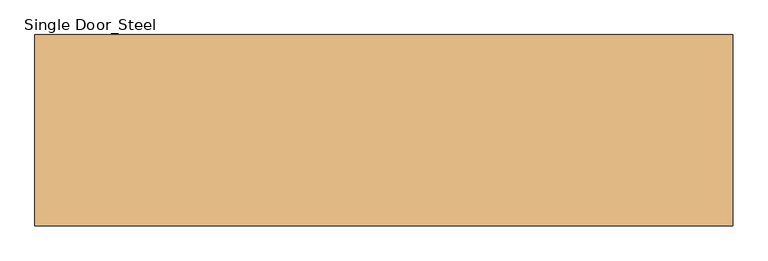
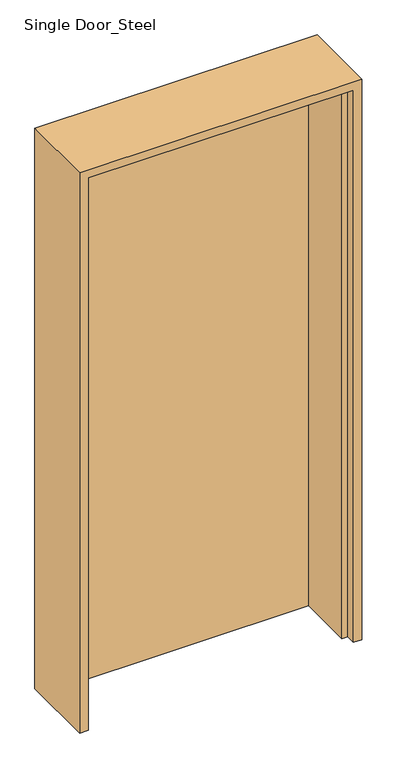
"""IFC4 building model written with IfcOpenShell, lengths in millimetres: door geometry, Single Door_Steel : H_DR_AMD_Single Door_Int_Steel_1000x2100."""

import ifcopenshell
import ifcopenshell.guid

model = None  # the IFC model being written
_history = None  # IfcOwnerHistory: only IFC2X3 demands one
_inside = {}  # id of a spatial element -> (the spatial element, [elements in it])
_under = {}  # id of a project, library or spatial element -> (it, [spatial elements below it])
_declared = {}  # id of a project -> (the project, [libraries it declares])
_typed = {}  # id of a type object -> (the type object, [elements of that type])
_made_of = {}  # id of a material, layer set ... -> (it, [elements and type objects made of it])


def new_model(schema):
    """Start an empty IFC model of exactly this schema.

    Asked for "IFC4X3", IfcOpenShell would pick the latest addendum, in which some entities
    have other attributes; the version numbers below select the first issue.
    IFC2X3 requires an IfcOwnerHistory on every rooted entity: one is made here for all.
    """
    global model, _history
    if schema == "IFC4X3":
        model = ifcopenshell.file(schema_version=(4, 3, 0, 0))
    else:
        model = ifcopenshell.file(schema=schema)
    _inside.clear()
    _under.clear()
    _declared.clear()
    _typed.clear()
    _made_of.clear()
    _history = None
    if model.schema == "IFC2X3":
        org = make("IfcOrganization", Name="unknown")
        user = make(
            "IfcPersonAndOrganization",
            ThePerson=make("IfcPerson", FamilyName="unknown"),
            TheOrganization=org,
        )
        app = make(
            "IfcApplication",
            ApplicationDeveloper=org,
            Version="unknown",
            ApplicationFullName="unknown",
            ApplicationIdentifier="unknown",
        )
        _history = make(
            "IfcOwnerHistory",
            OwningUser=user,
            OwningApplication=app,
            ChangeAction="ADDED",
            CreationDate=0,
        )
    return model


def make(cls, **values):
    """One entity of the class cls with the attributes given. An attribute that is None is left unset."""
    return model.create_entity(
        cls, **{name: value for name, value in values.items() if value is not None}
    )


def rooted(cls, **values):
    """An entity with a GlobalId (a new one), such as an element, a storey or a relation."""
    return make(cls, GlobalId=ifcopenshell.guid.new(), OwnerHistory=_history, **values)


def si_unit(unit_type, name, prefix=None):
    """IfcSIUnit, for example si_unit("LENGTHUNIT", "METRE", prefix="MILLI")."""
    return make("IfcSIUnit", UnitType=unit_type, Prefix=prefix, Name=name)


def assignment(units):
    """IfcUnitAssignment: the units of a project."""
    return None if units is None else make("IfcUnitAssignment", Units=units)


def point(xyz):
    """IfcCartesianPoint."""
    return None if xyz is None else make("IfcCartesianPoint", Coordinates=xyz)


def direction(xyz):
    """IfcDirection."""
    return None if xyz is None else make("IfcDirection", DirectionRatios=xyz)


def frame(location, z_axis=None, x_axis=None):
    """IfcAxis2Placement3D, a coordinate frame: its origin and axes. An axis left out is left unset."""
    return make(
        "IfcAxis2Placement3D",
        Location=point(location),
        Axis=direction(z_axis),
        RefDirection=direction(x_axis),
    )


def origin():
    """The frame at (0, 0, 0) with its axes left unset."""
    return frame((0.0, 0.0, 0.0))


def origin_with_axes():
    """The frame at (0, 0, 0) with the z axis (0, 0, 1) and the x axis (1, 0, 0) written out."""
    return frame((0.0, 0.0, 0.0), z_axis=(0.0, 0.0, 1.0), x_axis=(1.0, 0.0, 0.0))


def place(relative_to, where):
    """IfcLocalPlacement: puts the frame where relative to a parent placement (None: the world)."""
    return make(
        "IfcLocalPlacement", PlacementRelTo=relative_to, RelativePlacement=where
    )


def context(
    kind, dimensions, precision=None, world=None, true_north=None, identifier=None
):
    """IfcGeometricRepresentationContext, for example the 3D "Model" context."""
    return make(
        "IfcGeometricRepresentationContext",
        ContextIdentifier=identifier,
        ContextType=kind,
        CoordinateSpaceDimension=dimensions,
        Precision=precision,
        WorldCoordinateSystem=world,
        TrueNorth=true_north,
    )


def project(units=None, contexts=None):
    """IfcProject with its units and contexts."""
    return rooted(
        "IfcProject",
        Name="project",
        RepresentationContexts=contexts,
        UnitsInContext=assignment(units),
    )


def spatial(cls, under=None, at=None, **own):
    """A site, building, storey or space (cls), placed at a placement, below another one or the project."""
    s = rooted(cls, ObjectPlacement=at, **own)
    if under is not None:
        _under.setdefault(under.id(), (under, []))[1].append(s)
    return s


def polyline(points):
    """IfcPolyline through the points."""
    return make("IfcPolyline", Points=[point(p) for p in points])


def outline(outer, holes=None, kind="AREA"):
    """IfcArbitraryClosedProfileDef: a profile drawn as a closed curve; with holes, ...WithVoids."""
    if holes is None:
        return make("IfcArbitraryClosedProfileDef", ProfileType=kind, OuterCurve=outer)
    return make(
        "IfcArbitraryProfileDefWithVoids",
        ProfileType=kind,
        OuterCurve=outer,
        InnerCurves=holes,
    )


def extrude(swept, where, along, depth):
    """IfcExtrudedAreaSolid: the profile swept, set in the frame where, extruded along a direction by depth."""
    return make(
        "IfcExtrudedAreaSolid",
        SweptArea=swept,
        Position=where,
        ExtrudedDirection=direction(along),
        Depth=depth,
    )


def faces_of(points, faces, orient=None, outer=None):
    """IfcFace entities. A face is a list of loops; a loop is a list of indices into points, from 0.

    orient and outer hold one flag for each loop. By default every Orientation is true, the
    first loop of a face is its IfcFaceOuterBound and the others are IfcFaceBound.
    """
    made = []
    for i, loops in enumerate(faces):
        bounds = []
        for j, loop in enumerate(loops):
            is_outer = j == 0 if outer is None else outer[i][j]
            bounds.append(
                make(
                    "IfcFaceOuterBound" if is_outer else "IfcFaceBound",
                    Bound=make("IfcPolyLoop", Polygon=[points[k] for k in loop]),
                    Orientation=True if orient is None else orient[i][j],
                )
            )
        made.append(make("IfcFace", Bounds=bounds))
    return made


def faceted_brep(points, faces, orient=None, outer=None, voids=None):
    """IfcFacetedBrep: a solid bounded by flat faces; with voids (closed shells), ...WithVoids."""
    shared = [point(p) for p in points]
    hull = make("IfcClosedShell", CfsFaces=faces_of(shared, faces, orient, outer))
    if voids is None:
        return make("IfcFacetedBrep", Outer=hull)
    return make(
        "IfcFacetedBrepWithVoids",
        Outer=hull,
        Voids=[
            make(cls, CfsFaces=faces_of(shared, fs, o, b)) for cls, fs, o, b in voids
        ],
    )


def shape(context_of_items, identifier, shape_type, items):
    """IfcShapeRepresentation: the items that make up one representation, for example the "Body"."""
    return make(
        "IfcShapeRepresentation",
        ContextOfItems=context_of_items,
        RepresentationIdentifier=identifier,
        RepresentationType=shape_type,
        Items=items,
    )


def source(mapping_origin, context_of_items, identifier, shape_type, items):
    """IfcRepresentationMap: a shape defined once, which mapped items show again and again."""
    return make(
        "IfcRepresentationMap",
        MappingOrigin=mapping_origin,
        MappedRepresentation=shape(context_of_items, identifier, shape_type, items),
    )


def transform(
    local_origin,
    x_axis=None,
    y_axis=None,
    z_axis=None,
    scale=None,
    scale2=None,
    scale3=None,
    uniform=True,
):
    """IfcCartesianTransformationOperator3D, or its non-uniform kind. x_axis, y_axis, z_axis: its Axis1, 2, 3."""
    if uniform:
        return make(
            "IfcCartesianTransformationOperator3D",
            Axis1=direction(x_axis),
            Axis2=direction(y_axis),
            LocalOrigin=point(local_origin),
            Scale=scale,
            Axis3=direction(z_axis),
        )
    return make(
        "IfcCartesianTransformationOperator3DnonUniform",
        Axis1=direction(x_axis),
        Axis2=direction(y_axis),
        LocalOrigin=point(local_origin),
        Scale=scale,
        Axis3=direction(z_axis),
        Scale2=scale2,
        Scale3=scale3,
    )


def mapped(mapping_source, mapping_target):
    """IfcMappedItem: shows the shape of a source again, moved by a transform."""
    return make(
        "IfcMappedItem", MappingSource=mapping_source, MappingTarget=mapping_target
    )


def made_of(thing, what):
    """Note that an element or type object is made of a material, layer set ...; save() writes the relation."""
    if what is not None:
        _made_of.setdefault(what.id(), (what, []))[1].append(thing)
    return thing


def element(
    cls,
    number,
    at=None,
    inside=None,
    cuts=None,
    type_object=None,
    material=None,
    context=None,
    identifier="Body",
    shape_type=None,
    held_by="IfcProductDefinitionShape",
    body=None,
    shapes=None,
    **own,
):
    """One element of the class cls, such as IfcWall. Its Tag is "e" and its number.

    at: its placement. inside: the storey or other place that contains it. cuts: it is an
    opening in that element (IfcRelVoidsElement). A single representation is given by context,
    identifier, shape_type and body (its items); several are given by shapes. held_by: the class
    of the entity that holds the representations. save() writes the other relations.
    """
    e = rooted(cls, Tag="e%d" % number, ObjectPlacement=at, **own)
    if body is not None:
        shapes = [shape(context, identifier, shape_type, body)]
    if shapes is not None:
        e.Representation = make(held_by, Representations=shapes)
    if inside is not None:
        _inside.setdefault(inside.id(), (inside, []))[1].append(e)
    if cuts is not None:
        rooted(
            "IfcRelVoidsElement", RelatingBuildingElement=cuts, RelatedOpeningElement=e
        )
    if type_object is not None:
        _typed.setdefault(type_object.id(), (type_object, []))[1].append(e)
    return made_of(e, material)


def aggregate(whole, parts):
    """IfcRelAggregates: a whole, such as a stair, and the parts it consists of."""
    return rooted("IfcRelAggregates", RelatingObject=whole, RelatedObjects=parts)


def save(model, path):
    """Write the relations noted so far, then the file.

    IfcRelAggregates (storeys below a building ...), IfcRelContainedInSpatialStructure (elements
    in a storey), IfcRelDefinesByType, IfcRelAssociatesMaterial and IfcRelDeclares: one each for
    every whole, place, type object, material and project.
    """
    for whole, parts in _under.values():
        aggregate(whole, parts)
    for where, things in _inside.values():
        rooted(
            "IfcRelContainedInSpatialStructure",
            RelatedElements=things,
            RelatingStructure=where,
        )
    for kind, things in _typed.values():
        rooted("IfcRelDefinesByType", RelatedObjects=things, RelatingType=kind)
    for what, things in _made_of.values():
        rooted("IfcRelAssociatesMaterial", RelatedObjects=things, RelatingMaterial=what)
    for by, libraries in _declared.values():
        rooted("IfcRelDeclares", RelatingContext=by, RelatedDefinitions=libraries)
    model.write(path)


def single_door_steel_d0b51d4b(model_context):
    return source(origin(), model_context, "Body", "SolidModel", [
        extrude(outline(polyline([(470.0, 137.0), (470.0, 102.0), (-470.0, 102.0), (-470.0, 137.0), (470.0, 137.0)])), origin_with_axes(), (0.0, 0.0, 1.0), 2070.0),
        faceted_brep([(470.0, 137.0, 0.0), (500.0, 137.0, 0.0), (500.0, -137.0, 0.0), (470.0, -137.0, 0.0), (470.0, -102.0, 0.0), (450.0, -102.0, 0.0), (450.0, 102.0, 0.0), (470.0, 102.0, 0.0), (470.0, 137.0, 2070.0), (-470.0, 137.0, 2070.0), (-470.0, 137.0, 0.0), (-500.0, 137.0, 0.0), (-500.0, 137.0, 2100.0), (500.0, 137.0, 2100.0), (500.0, -137.0, 2100.0), (-500.0, -137.0, 2100.0), (-500.0, -137.0, 0.0), (-470.0, -137.0, 0.0), (-470.0, -137.0, 2070.0), (470.0, -137.0, 2070.0), (470.0, -102.0, 2070.0), (-470.0, -102.0, 2070.0), (-470.0, -102.0, 0.0), (-450.0, -102.0, 0.0), (-450.0, -102.0, 2050.0), (450.0, -102.0, 2050.0), (450.0, 102.0, 2050.0), (-450.0, 102.0, 2050.0), (-450.0, 102.0, 0.0), (-470.0, 102.0, 0.0), (-470.0, 102.0, 2070.0), (470.0, 102.0, 2070.0)], [[[0, 1, 2, 3, 4, 5, 6, 7]], [[1, 0, 8, 9, 10, 11, 12, 13]], [[2, 1, 13, 14]], [[3, 2, 14, 15, 16, 17, 18, 19]], [[4, 3, 19, 20]], [[5, 4, 20, 21, 22, 23, 24, 25]], [[6, 5, 25, 26]], [[7, 6, 26, 27, 28, 29, 30, 31]], [[0, 7, 31, 8]], [[9, 30, 29, 10]], [[10, 29, 28, 23, 22, 17, 16, 11]], [[15, 12, 11, 16]], [[21, 18, 17, 22]], [[27, 24, 23, 28]], [[14, 13, 12, 15]], [[20, 19, 18, 21]], [[26, 25, 24, 27]], [[8, 31, 30, 9]]]),
    ])


if __name__ == "__main__":
    model = new_model("IFC4")
    model_context = context("Model", 3, world=origin())
    ifc_project = project(units=[si_unit("LENGTHUNIT", "METRE", prefix="MILLI")], contexts=[model_context])
    site = spatial("IfcSite", under=ifc_project)
    building = spatial("IfcBuilding", under=site)
    placement = place(None, origin())
    single_door_steel_shape = single_door_steel_d0b51d4b(model_context)
    element("IfcDoor", 1, ObjectType="Single Door_Steel : H_DR_AMD_Single Door_Int_Steel_1000x2100", at=placement, inside=building, context=model_context, shape_type="MappedRepresentation", body=[
        mapped(single_door_steel_shape, transform((0.0, 0.0, 0.0), x_axis=(1.0, 0.0, 0.0), y_axis=(0.0, 1.0, 0.0), z_axis=(0.0, 0.0, 1.0))),
    ])
    save(model, "model.ifc")

# Revit data of these elements
# Type "Single Door_Steel : H_DR_AMD_Single Door_Int_Steel_1000x2100"
#   Type Mark = "SD"
#   Analytic Construction = "<None>"
#   프레임 투영 외부. = 0.0250 m
#   프레임 투영 내부. = 0.0250 m
#   프레임 폭 = 0.0750 m
#   Height = 2.1000 m
#   Width = 1.0000 m
#   Define Thermal Properties by = 1
#   문 패널 = SD1 문 패널
#   문 프레임 = A04AR099-00001_Steel Door_Single_FR_N
#   Function = (empty or 0)
#   Wall Closure = (empty or 0)
# Element 1 (IfcDoor, "Single Door_Steel : H_DR_AMD_Single Door_Int_Steel_1000x2100")
#   Materials on its faces: "A04AR099-00001_Steel Door_Single_FR_N", "SD1 문 패널"
# Materials
#   "SD1 문 패널": class "금속", colour RGB 247 247 247, transparency 0, Description = "STEEL DOOR (1000Wx2100H)"
#   "A04AR099-00001_Steel Door_Single_FR_N": class "Metal", colour RGB 247 247 247, transparency 0, Description = "Steel Door w/ Steel Frame", Cost = 0
